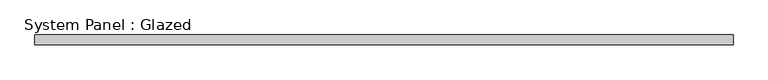
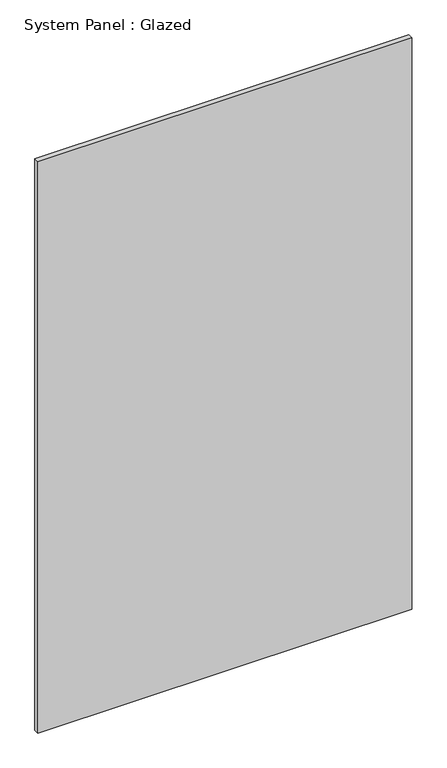
"""IFC4 building model written with IfcOpenShell, lengths in millimetres: plate geometry, System Panel : Glazed."""

from ifc_helpers import new_model, si_unit, origin, origin_with_axes, place, context, project, spatial, polyline, outline, extrude, source, transform, mapped, element, save


def system_panel_glazed_306e4401(model_context):
    return source(origin(), model_context, "Body", "SweptSolid", [
        extrude(outline(polyline([(905.5833335, 24.5), (-905.5833335, 24.5), (-905.5833335, 49.5), (905.5833335, 49.5), (905.5833335, 24.5)])), origin_with_axes(), (0.0, 0.0, 1.0), 2925.0),
    ])


if __name__ == "__main__":
    model = new_model("IFC4")
    model_context = context("Model", 3, world=origin())
    ifc_project = project(units=[si_unit("LENGTHUNIT", "METRE", prefix="MILLI")], contexts=[model_context])
    site = spatial("IfcSite", under=ifc_project)
    building = spatial("IfcBuilding", under=site)
    placement = place(None, origin())
    system_panel_glazed_shape = system_panel_glazed_306e4401(model_context)
    element("IfcPlate", 1, ObjectType="System Panel : Glazed", at=placement, inside=building, context=model_context, shape_type="MappedRepresentation", body=[
        mapped(system_panel_glazed_shape, transform((0.0, 0.0, 0.0), x_axis=(1.0, 0.0, 0.0), y_axis=(0.0, 1.0, 0.0), z_axis=(0.0, 0.0, 1.0))),
    ])
    save(model, "model.ifc")

# Revit data of these elements
# Element 1 (IfcPlate, "System Panel : Glazed")
#   Materials on its faces: "Glass"
# Materials
#   "Glass": class "Glass", colour RGB 0 128 192, transparency 0.9
